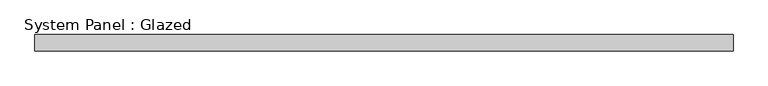
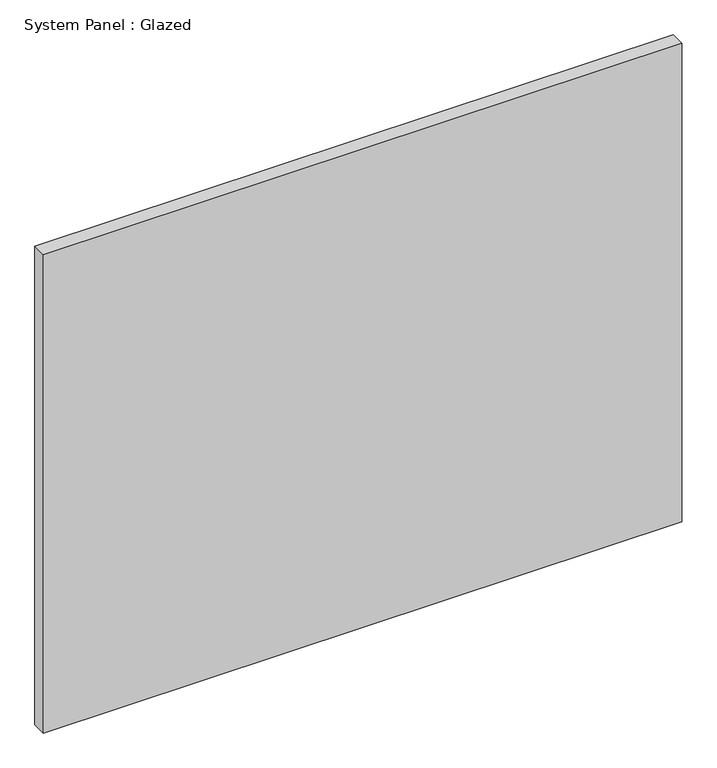
"""IFC4 building model written with IfcOpenShell, lengths in millimetres: plate geometry, System Panel : Glazed."""

from ifc_helpers import new_model, si_unit, origin, origin_with_axes, place, context, project, spatial, polyline, outline, extrude, source, transform, mapped, element, save


def system_panel_glazed_8c2c847a(model_context):
    return source(origin(), model_context, "Body", "SweptSolid", [
        extrude(outline(polyline([(549.275, 19.05), (-549.275, 19.05), (-549.275, 44.45), (549.275, 44.45), (549.275, 19.05)])), origin_with_axes(), (0.0, 0.0, 1.0), 869.95),
    ])


if __name__ == "__main__":
    model = new_model("IFC4")
    model_context = context("Model", 3, world=origin())
    ifc_project = project(units=[si_unit("LENGTHUNIT", "METRE", prefix="MILLI")], contexts=[model_context])
    site = spatial("IfcSite", under=ifc_project)
    building = spatial("IfcBuilding", under=site)
    placement = place(None, origin())
    system_panel_glazed_shape = system_panel_glazed_8c2c847a(model_context)
    element("IfcPlate", 1, ObjectType="System Panel : Glazed", at=placement, inside=building, context=model_context, shape_type="MappedRepresentation", body=[
        mapped(system_panel_glazed_shape, transform((0.0, 0.0, 0.0), x_axis=(1.0, 0.0, 0.0), y_axis=(0.0, 1.0, 0.0), z_axis=(0.0, 0.0, 1.0))),
    ])
    save(model, "model.ifc")

# Revit data of these elements
# Element 1 (IfcPlate, "System Panel : Glazed")
#   Materials on its faces: "Glass"
# Materials
#   "Glass": class "Glass", colour RGB 0 128 192, transparency 0.75
